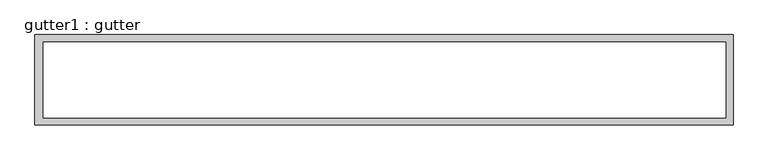
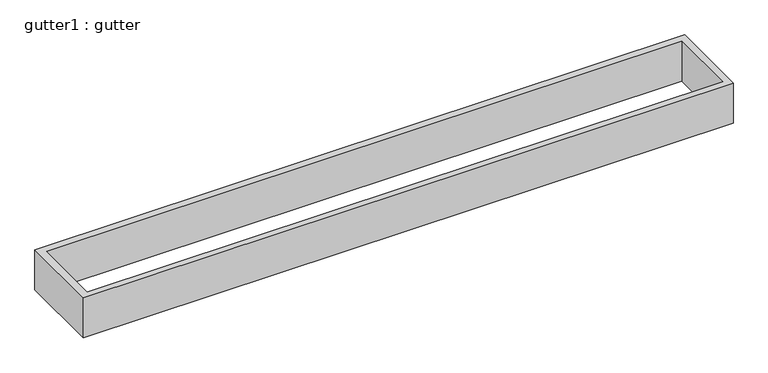
"""IFC4 building model written with IfcOpenShell, lengths in millimetres: proxy geometry, gutter1 : gutter."""

from ifc_helpers import new_model, si_unit, frame, origin, place, context, project, spatial, polyline, outline, extrude, source, transform, mapped, element, save


def gutter1_gutter_22c69523(model_context):
    return source(origin(), model_context, "Body", "SweptSolid", [
        extrude(outline(polyline([(29665.9107095, 1909.5502616), (24977.1521553, 1909.5502616), (24977.1521553, 2515.8615366), (29665.9107095, 2515.8615366), (29665.9107095, 1909.5502616)]), holes=[polyline([(29616.401408, 2465.0615366), (25031.5521553, 2465.0615366), (25031.5521553, 1956.0872459), (29616.401408, 1956.0872459), (29616.401408, 2465.0615366)])]), frame((0.0, 0.0, 2832.1), z_axis=(0.0, 0.0, 1.0), x_axis=(1.0, 0.0, 0.0)), (0.0, 0.0, 1.0), 304.8),
    ])


if __name__ == "__main__":
    model = new_model("IFC4")
    model_context = context("Model", 3, world=origin())
    ifc_project = project(units=[si_unit("LENGTHUNIT", "METRE", prefix="MILLI")], contexts=[model_context])
    site = spatial("IfcSite", under=ifc_project)
    building = spatial("IfcBuilding", under=site)
    placement = place(None, origin())
    gutter1_gutter_shape = gutter1_gutter_22c69523(model_context)
    element("IfcBuildingElementProxy", 1, Name="gutter1 : gutter", ObjectType="gutter1 : gutter", at=placement, inside=building, context=model_context, shape_type="MappedRepresentation", body=[
        mapped(gutter1_gutter_shape, transform((0.0, 0.0, 0.0), x_axis=(1.0, 0.0, 0.0), y_axis=(0.0, 1.0, 0.0), z_axis=(0.0, 0.0, 1.0))),
    ])
    save(model, "model.ifc")
